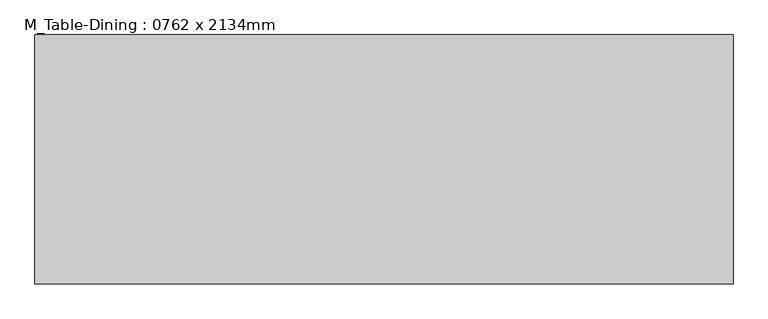
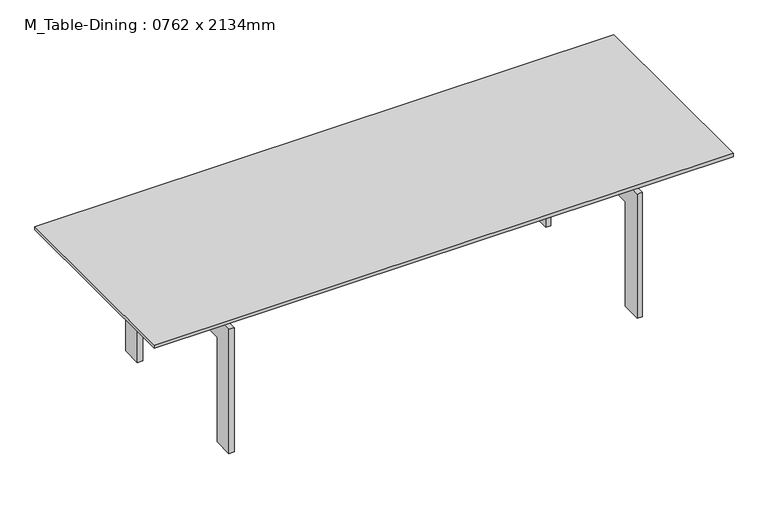
"""IFC4 building model written with IfcOpenShell, lengths in millimetres: furniture geometry, M_Table-Dining : 0762 x 2134mm."""

import ifcopenshell
import ifcopenshell.guid

model = None  # the IFC model being written
_history = None  # IfcOwnerHistory: only IFC2X3 demands one
_inside = {}  # id of a spatial element -> (the spatial element, [elements in it])
_under = {}  # id of a project, library or spatial element -> (it, [spatial elements below it])
_declared = {}  # id of a project -> (the project, [libraries it declares])
_typed = {}  # id of a type object -> (the type object, [elements of that type])
_made_of = {}  # id of a material, layer set ... -> (it, [elements and type objects made of it])


def new_model(schema):
    """Start an empty IFC model of exactly this schema.

    Asked for "IFC4X3", IfcOpenShell would pick the latest addendum, in which some entities
    have other attributes; the version numbers below select the first issue.
    IFC2X3 requires an IfcOwnerHistory on every rooted entity: one is made here for all.
    """
    global model, _history
    if schema == "IFC4X3":
        model = ifcopenshell.file(schema_version=(4, 3, 0, 0))
    else:
        model = ifcopenshell.file(schema=schema)
    _inside.clear()
    _under.clear()
    _declared.clear()
    _typed.clear()
    _made_of.clear()
    _history = None
    if model.schema == "IFC2X3":
        org = make("IfcOrganization", Name="unknown")
        user = make(
            "IfcPersonAndOrganization",
            ThePerson=make("IfcPerson", FamilyName="unknown"),
            TheOrganization=org,
        )
        app = make(
            "IfcApplication",
            ApplicationDeveloper=org,
            Version="unknown",
            ApplicationFullName="unknown",
            ApplicationIdentifier="unknown",
        )
        _history = make(
            "IfcOwnerHistory",
            OwningUser=user,
            OwningApplication=app,
            ChangeAction="ADDED",
            CreationDate=0,
        )
    return model


def make(cls, **values):
    """One entity of the class cls with the attributes given. An attribute that is None is left unset."""
    return model.create_entity(
        cls, **{name: value for name, value in values.items() if value is not None}
    )


def rooted(cls, **values):
    """An entity with a GlobalId (a new one), such as an element, a storey or a relation."""
    return make(cls, GlobalId=ifcopenshell.guid.new(), OwnerHistory=_history, **values)


def si_unit(unit_type, name, prefix=None):
    """IfcSIUnit, for example si_unit("LENGTHUNIT", "METRE", prefix="MILLI")."""
    return make("IfcSIUnit", UnitType=unit_type, Prefix=prefix, Name=name)


def assignment(units):
    """IfcUnitAssignment: the units of a project."""
    return None if units is None else make("IfcUnitAssignment", Units=units)


def point(xyz):
    """IfcCartesianPoint."""
    return None if xyz is None else make("IfcCartesianPoint", Coordinates=xyz)


def direction(xyz):
    """IfcDirection."""
    return None if xyz is None else make("IfcDirection", DirectionRatios=xyz)


def frame(location, z_axis=None, x_axis=None):
    """IfcAxis2Placement3D, a coordinate frame: its origin and axes. An axis left out is left unset."""
    return make(
        "IfcAxis2Placement3D",
        Location=point(location),
        Axis=direction(z_axis),
        RefDirection=direction(x_axis),
    )


def origin():
    """The frame at (0, 0, 0) with its axes left unset."""
    return frame((0.0, 0.0, 0.0))


def place(relative_to, where):
    """IfcLocalPlacement: puts the frame where relative to a parent placement (None: the world)."""
    return make(
        "IfcLocalPlacement", PlacementRelTo=relative_to, RelativePlacement=where
    )


def context(
    kind, dimensions, precision=None, world=None, true_north=None, identifier=None
):
    """IfcGeometricRepresentationContext, for example the 3D "Model" context."""
    return make(
        "IfcGeometricRepresentationContext",
        ContextIdentifier=identifier,
        ContextType=kind,
        CoordinateSpaceDimension=dimensions,
        Precision=precision,
        WorldCoordinateSystem=world,
        TrueNorth=true_north,
    )


def project(units=None, contexts=None):
    """IfcProject with its units and contexts."""
    return rooted(
        "IfcProject",
        Name="project",
        RepresentationContexts=contexts,
        UnitsInContext=assignment(units),
    )


def spatial(cls, under=None, at=None, **own):
    """A site, building, storey or space (cls), placed at a placement, below another one or the project."""
    s = rooted(cls, ObjectPlacement=at, **own)
    if under is not None:
        _under.setdefault(under.id(), (under, []))[1].append(s)
    return s


def polyline(points):
    """IfcPolyline through the points."""
    return make("IfcPolyline", Points=[point(p) for p in points])


def outline(outer, holes=None, kind="AREA"):
    """IfcArbitraryClosedProfileDef: a profile drawn as a closed curve; with holes, ...WithVoids."""
    if holes is None:
        return make("IfcArbitraryClosedProfileDef", ProfileType=kind, OuterCurve=outer)
    return make(
        "IfcArbitraryProfileDefWithVoids",
        ProfileType=kind,
        OuterCurve=outer,
        InnerCurves=holes,
    )


def extrude(swept, where, along, depth):
    """IfcExtrudedAreaSolid: the profile swept, set in the frame where, extruded along a direction by depth."""
    return make(
        "IfcExtrudedAreaSolid",
        SweptArea=swept,
        Position=where,
        ExtrudedDirection=direction(along),
        Depth=depth,
    )


def shape(context_of_items, identifier, shape_type, items):
    """IfcShapeRepresentation: the items that make up one representation, for example the "Body"."""
    return make(
        "IfcShapeRepresentation",
        ContextOfItems=context_of_items,
        RepresentationIdentifier=identifier,
        RepresentationType=shape_type,
        Items=items,
    )


def source(mapping_origin, context_of_items, identifier, shape_type, items):
    """IfcRepresentationMap: a shape defined once, which mapped items show again and again."""
    return make(
        "IfcRepresentationMap",
        MappingOrigin=mapping_origin,
        MappedRepresentation=shape(context_of_items, identifier, shape_type, items),
    )


def transform(
    local_origin,
    x_axis=None,
    y_axis=None,
    z_axis=None,
    scale=None,
    scale2=None,
    scale3=None,
    uniform=True,
):
    """IfcCartesianTransformationOperator3D, or its non-uniform kind. x_axis, y_axis, z_axis: its Axis1, 2, 3."""
    if uniform:
        return make(
            "IfcCartesianTransformationOperator3D",
            Axis1=direction(x_axis),
            Axis2=direction(y_axis),
            LocalOrigin=point(local_origin),
            Scale=scale,
            Axis3=direction(z_axis),
        )
    return make(
        "IfcCartesianTransformationOperator3DnonUniform",
        Axis1=direction(x_axis),
        Axis2=direction(y_axis),
        LocalOrigin=point(local_origin),
        Scale=scale,
        Axis3=direction(z_axis),
        Scale2=scale2,
        Scale3=scale3,
    )


def mapped(mapping_source, mapping_target):
    """IfcMappedItem: shows the shape of a source again, moved by a transform."""
    return make(
        "IfcMappedItem", MappingSource=mapping_source, MappingTarget=mapping_target
    )


def made_of(thing, what):
    """Note that an element or type object is made of a material, layer set ...; save() writes the relation."""
    if what is not None:
        _made_of.setdefault(what.id(), (what, []))[1].append(thing)
    return thing


def element(
    cls,
    number,
    at=None,
    inside=None,
    cuts=None,
    type_object=None,
    material=None,
    context=None,
    identifier="Body",
    shape_type=None,
    held_by="IfcProductDefinitionShape",
    body=None,
    shapes=None,
    **own,
):
    """One element of the class cls, such as IfcWall. Its Tag is "e" and its number.

    at: its placement. inside: the storey or other place that contains it. cuts: it is an
    opening in that element (IfcRelVoidsElement). A single representation is given by context,
    identifier, shape_type and body (its items); several are given by shapes. held_by: the class
    of the entity that holds the representations. save() writes the other relations.
    """
    e = rooted(cls, Tag="e%d" % number, ObjectPlacement=at, **own)
    if body is not None:
        shapes = [shape(context, identifier, shape_type, body)]
    if shapes is not None:
        e.Representation = make(held_by, Representations=shapes)
    if inside is not None:
        _inside.setdefault(inside.id(), (inside, []))[1].append(e)
    if cuts is not None:
        rooted(
            "IfcRelVoidsElement", RelatingBuildingElement=cuts, RelatedOpeningElement=e
        )
    if type_object is not None:
        _typed.setdefault(type_object.id(), (type_object, []))[1].append(e)
    return made_of(e, material)


def aggregate(whole, parts):
    """IfcRelAggregates: a whole, such as a stair, and the parts it consists of."""
    return rooted("IfcRelAggregates", RelatingObject=whole, RelatedObjects=parts)


def save(model, path):
    """Write the relations noted so far, then the file.

    IfcRelAggregates (storeys below a building ...), IfcRelContainedInSpatialStructure (elements
    in a storey), IfcRelDefinesByType, IfcRelAssociatesMaterial and IfcRelDeclares: one each for
    every whole, place, type object, material and project.
    """
    for whole, parts in _under.values():
        aggregate(whole, parts)
    for where, things in _inside.values():
        rooted(
            "IfcRelContainedInSpatialStructure",
            RelatedElements=things,
            RelatingStructure=where,
        )
    for kind, things in _typed.values():
        rooted("IfcRelDefinesByType", RelatedObjects=things, RelatingType=kind)
    for what, things in _made_of.values():
        rooted("IfcRelAssociatesMaterial", RelatedObjects=things, RelatingMaterial=what)
    for by, libraries in _declared.values():
        rooted("IfcRelDeclares", RelatingContext=by, RelatedDefinitions=libraries)
    model.write(path)


def m_table_dining_0762_x_2134mm_3327233b(model_context):
    return source(origin(), model_context, "Body", "SweptSolid", [
        extrude(outline(polyline([(983.6657667, 297.7823857), (983.6657667, 272.3823857), (-947.1342333, 272.3823857), (-947.1342333, 297.7823857), (983.6657667, 297.7823857)])), frame((0.0, 0.0, 483.8), z_axis=(0.0, 0.0, 1.0), x_axis=(1.0, 0.0, 0.0)), (0.0, 0.0, 1.0), 63.5),
        extrude(outline(polyline([(983.6657667, -82.5889222), (983.6657667, -107.9889222), (-947.1342333, -107.9889222), (-947.1342333, -82.5889222), (983.6657667, -82.5889222)])), frame((0.0, 0.0, 483.8), z_axis=(0.0, 0.0, 1.0), x_axis=(1.0, 0.0, 0.0)), (0.0, 0.0, 1.0), 63.5),
        extrude(outline(polyline([(425.4110778, 0.0), (349.2110778, 0.0), (349.2110778, 407.6), (-158.7889222, 407.6), (-158.7889222, 0.0), (-234.9889222, 0.0), (-234.9889222, 483.8), (425.4110778, 483.8), (425.4110778, 0.0)])), frame((761.4157667, 0.0, 0.0), z_axis=(1.0, 0.0, 0.0), x_axis=(0.0, 1.0, 0.0)), (0.0, 0.0, 1.0), 19.05),
        extrude(outline(polyline([(425.4110778, 483.8), (425.4110778, 0.0), (349.2110778, 0.0), (349.2110778, 407.6), (-158.7889222, 407.6), (-158.7889222, 0.0), (-234.9889222, 0.0), (-234.9889222, 483.8), (425.4110778, 483.8)])), frame((-743.9342333, 0.0, 0.0), z_axis=(1.0, 0.0, 0.0), x_axis=(0.0, 1.0, 0.0)), (0.0, 0.0, 1.0), 19.05),
        extrude(outline(polyline([(1085.2657667, 476.2110778), (1085.2657667, -285.7889222), (-1048.7342333, -285.7889222), (-1048.7342333, 476.2110778), (1085.2657667, 476.2110778)])), frame((0.0, 0.0, 547.3), z_axis=(0.0, 0.0, 1.0), x_axis=(1.0, 0.0, 0.0)), (0.0, 0.0, 1.0), 12.7),
    ])


if __name__ == "__main__":
    model = new_model("IFC4")
    model_context = context("Model", 3, world=origin())
    ifc_project = project(units=[si_unit("LENGTHUNIT", "METRE", prefix="MILLI")], contexts=[model_context])
    site = spatial("IfcSite", under=ifc_project)
    building = spatial("IfcBuilding", under=site)
    placement = place(None, origin())
    m_table_dining_0762_x_2134mm_shape = m_table_dining_0762_x_2134mm_3327233b(model_context)
    element("IfcFurniture", 1, ObjectType="M_Table-Dining : 0762 x 2134mm", at=placement, inside=building, context=model_context, shape_type="MappedRepresentation", body=[
        mapped(m_table_dining_0762_x_2134mm_shape, transform((0.0, 0.0, 0.0), x_axis=(1.0, 0.0, 0.0), y_axis=(0.0, 1.0, 0.0), z_axis=(0.0, 0.0, 1.0))),
    ])
    save(model, "model.ifc")

# Revit data of these elements
# Type "M_Table-Dining : 0762 x 2134mm"
#   Height = 0.56 m
#   Length = 2.134 m
#   Width = 0.762 m
#   Base Material = Steel, Chrome Plated
#   Top Material = Glass - Clear, Grey
# Element 1 (IfcFurniture, "M_Table-Dining : 0762 x 2134mm")
#   Materials on its faces: "Steel, Chrome Plated", "Glass - Clear, Grey"
# Materials
#   "Steel, Chrome Plated": class "Metal", colour RGB 244 244 244, transparency 0, Description = "Chromiuim plated steel", Cost = 0
#   "Glass - Clear, Grey": class "Glass", colour RGB 252 255 255, transparency 0.64
